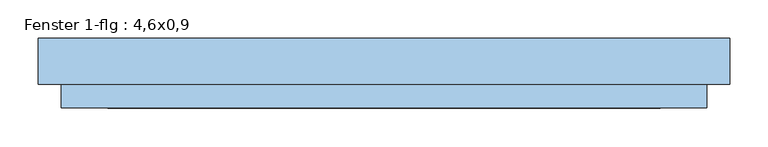
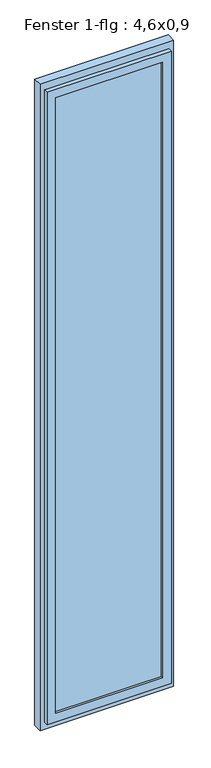
"""IFC4 building model written with IfcOpenShell, lengths in millimetres: window geometry, Fenster 1-flg : 4,6x0,9."""

from ifc_helpers import new_model, si_unit, frame, origin, place, context, project, spatial, polyline, outline, extrude, faceted_brep, source, transform, mapped, element, save


def fenster_1_flg_4_6x0_9_dbee532d(model_context):
    return source(origin(), model_context, "Body", "SolidModel", [
        extrude(outline(polyline([(5600.0, 450.0), (5600.0, -450.0), (1000.0, -450.0), (1000.0, 450.0), (5600.0, 450.0)]), holes=[polyline([(5520.0, 390.0), (1080.0, 390.0), (1080.0, -390.0), (5520.0, -390.0), (5520.0, 390.0)])]), frame((0.0, 20.0, 0.0), z_axis=(0.0, 1.0, 0.0), x_axis=(0.0, 0.0, 1.0)), (0.0, 0.0, 1.0), 60.0),
        faceted_brep([(420.0, 20.0, 5550.0), (420.0, -10.0, 5550.0), (420.0, -10.0, 1050.0), (420.0, 20.0, 1050.0), (-420.0, -10.0, 5550.0), (-420.0, -10.0, 1050.0), (360.0, -10.0, 1110.0), (-360.0, -10.0, 1110.0), (-360.0, -10.0, 5490.0), (360.0, -10.0, 5490.0), (-420.0, 20.0, 1050.0), (-420.0, 20.0, 5550.0), (390.0, 20.0, 5520.0), (-390.0, 20.0, 5520.0), (-390.0, 20.0, 1080.0), (390.0, 20.0, 1080.0), (390.0, 50.0, 5520.0), (390.0, 50.0, 1080.0), (-390.0, 50.0, 1080.0), (-390.0, 50.0, 5520.0), (360.0, 50.0, 5490.0), (-360.0, 50.0, 5490.0), (-360.0, 50.0, 1110.0), (360.0, 50.0, 1110.0)], [[[0, 1, 2, 3]], [[1, 4, 5, 2], [6, 7, 8, 9]], [[3, 2, 5, 10]], [[3, 10, 11, 0], [12, 13, 14, 15]], [[16, 12, 15, 17]], [[17, 15, 14, 18]], [[17, 18, 19, 16], [20, 21, 22, 23]], [[9, 20, 23, 6]], [[6, 23, 22, 7]], [[10, 5, 4, 11]], [[18, 14, 13, 19]], [[7, 22, 21, 8]], [[11, 4, 1, 0]], [[19, 13, 12, 16]], [[8, 21, 20, 9]]]),
        extrude(outline(polyline([(360.0, 5.0), (-360.0, 5.0), (-360.0, 35.0), (360.0, 35.0), (360.0, 5.0)])), frame((0.0, 0.0, 1110.0), z_axis=(0.0, 0.0, 1.0), x_axis=(1.0, 0.0, 0.0)), (0.0, 0.0, 1.0), 4380.0),
    ])


if __name__ == "__main__":
    model = new_model("IFC4")
    model_context = context("Model", 3, world=origin())
    ifc_project = project(units=[si_unit("LENGTHUNIT", "METRE", prefix="MILLI")], contexts=[model_context])
    site = spatial("IfcSite", under=ifc_project)
    building = spatial("IfcBuilding", under=site)
    placement = place(None, origin())
    fenster_1_flg_4_6x0_9_shape = fenster_1_flg_4_6x0_9_dbee532d(model_context)
    element("IfcWindow", 1, ObjectType="Fenster 1-flg : 4,6x0,9", at=placement, inside=building, context=model_context, shape_type="MappedRepresentation", body=[
        mapped(fenster_1_flg_4_6x0_9_shape, transform((0.0, 0.0, 0.0), x_axis=(1.0, 0.0, 0.0), y_axis=(0.0, 1.0, 0.0), z_axis=(0.0, 0.0, 1.0))),
    ])
    save(model, "model.ifc")

# Revit data of these elements
# Type "Fenster 1-flg : 4,6x0,9"
#   Type Mark = "60"
#   Operation = "SinglePanel"
#   Keynote = "16.05.01"
#   Visual Light Transmittance = 0.9
#   Solar Heat Gain Coefficient = 0.86
#   Rough Width = 0.900 m
#   Rough Height = 4.600 m
#   Heat Transfer Coefficient (U) = 5.5617 W/(m²·K)
#   Rahmentiefe = 0.060 m
#   Rahmenhöhe - unten = 0.080 m
#   Rahmenhöhe - oben = 0.080 m
#   Rahmenbreite = 0.060 m
#   Height = 4.600 m
#   Tiefe Flügel = 0.060 m
#   Flügelbreite = 0.060 m
#   Einbautiefe (von außen) [instance default] = 0.100 m
#   Width = 0.900 m
#   Klappflügel [instance default] = no
#   Kippflügel [instance default] = yes
#   Öffnungsrichtung in Draufsicht anzeigen [instance default] = no
#   Drehflügel 1 [instance default] = yes
#   Rahmen 1 [instance default] = none
#   Glas [instance default] = none
#   Flügel [instance default] = none
#   Fensterbank Innenseite [instance default] = none
#   Fensterbank Außenseite [instance default] = none
#   Construction Type Id = ""
#   Wall Closure = (empty or 0)
#   Analytic Construction = (empty or 0)
# Element 1 (IfcWindow, "Fenster 1-flg : 4,6x0,9")
#   Einbautiefe (von außen) = 0.230 m
#   Materials on its faces: "Kunststoff - Weiß", "Glas"
# Materials
#   "Kunststoff - Weiß": class "Kunststoff", colour RGB 249 249 249, transparency 0, Cost = 0
#   "Glas": class "Glas", colour RGB 0 0 255, transparency 0.75, Comments = "Render-Darstellung nicht aktualisiert ", Cost = 0
